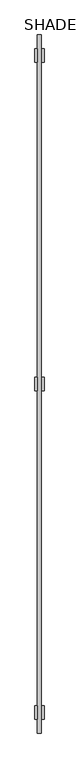
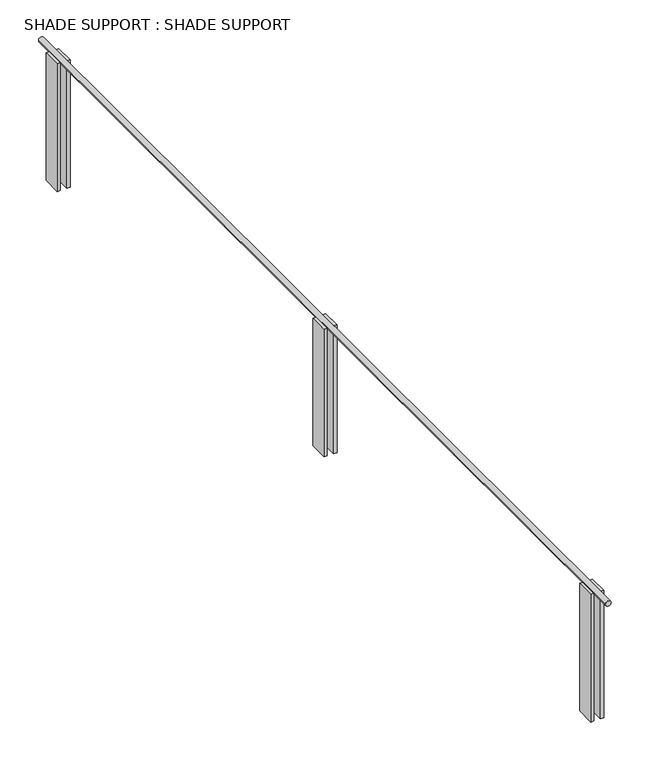
"""IFC4 building model written with IfcOpenShell, lengths in millimetres: proxy geometry, SHADE SUPPORT : SHADE SUPPORT."""

from ifc_helpers import new_model, si_unit, point, frame, frame_2d, origin, origin_with_axes, place, context, project, spatial, polyline, circle_curve, trimmed, segment, composite_curve, outline, extrude, source, transform, mapped, element, save


def shade_support_shade_support_fc9bf8e5(model_context):
    return source(origin(), model_context, "Body", "SweptSolid", [
        extrude(outline(composite_curve([segment(trimmed(circle_curve(frame_2d((1066.8, 0.0)), 22.225), [point((1066.8, -22.225))], [point((1066.8, 22.225))], False, "CARTESIAN"), True, "CONTINUOUS"), segment(trimmed(circle_curve(frame_2d((1066.8, 0.0)), 22.225), [point((1066.8, 22.225))], [point((1066.8, -22.225))], False, "CARTESIAN"), True, "CONTINUOUS")], self_intersect=False)), frame((0.0, -304.8, 0.0), z_axis=(0.0, 1.0, 0.0), x_axis=(0.0, 0.0, 1.0)), (0.0, 0.0, 1.0), 7772.4),
        extrude(outline(polyline([(-25.4, -152.4), (-50.8, -152.4), (-50.8, 0.0), (-25.4, 0.0), (-25.4, -152.4)])), origin_with_axes(), (0.0, 0.0, 1.0), 1066.8),
        extrude(outline(polyline([(50.8, -152.4), (25.4, -152.4), (25.4, 0.0), (50.8, 0.0), (50.8, -152.4)])), origin_with_axes(), (0.0, 0.0, 1.0), 1066.8),
        extrude(outline(polyline([(50.8, 3505.2), (25.4, 3505.2), (25.4, 3657.6), (50.8, 3657.6), (50.8, 3505.2)])), origin_with_axes(), (0.0, 0.0, 1.0), 1066.8),
        extrude(outline(polyline([(-25.4, 3505.2), (-50.8, 3505.2), (-50.8, 3657.6), (-25.4, 3657.6), (-25.4, 3505.2)])), origin_with_axes(), (0.0, 0.0, 1.0), 1066.8),
        extrude(outline(polyline([(50.8, 7162.8), (25.4, 7162.8), (25.4, 7315.2), (50.8, 7315.2), (50.8, 7162.8)])), origin_with_axes(), (0.0, 0.0, 1.0), 1066.8),
        extrude(outline(polyline([(-25.4, 7162.8), (-50.8, 7162.8), (-50.8, 7315.2), (-25.4, 7315.2), (-25.4, 7162.8)])), origin_with_axes(), (0.0, 0.0, 1.0), 1066.8),
    ])


if __name__ == "__main__":
    model = new_model("IFC4")
    model_context = context("Model", 3, world=origin())
    ifc_project = project(units=[si_unit("LENGTHUNIT", "METRE", prefix="MILLI")], contexts=[model_context])
    site = spatial("IfcSite", under=ifc_project)
    building = spatial("IfcBuilding", under=site)
    placement = place(None, origin())
    shade_support_shade_support_shape = shade_support_shade_support_fc9bf8e5(model_context)
    element("IfcBuildingElementProxy", 1, Name="SHADE SUPPORT : SHADE SUPPORT", ObjectType="SHADE SUPPORT : SHADE SUPPORT", at=placement, inside=building, context=model_context, shape_type="MappedRepresentation", body=[
        mapped(shade_support_shade_support_shape, transform((0.0, 0.0, 0.0), x_axis=(1.0, 0.0, 0.0), y_axis=(0.0, 1.0, 0.0), z_axis=(0.0, 0.0, 1.0))),
    ])
    save(model, "model.ifc")

# Revit data of these elements
# Type "SHADE SUPPORT : SHADE SUPPORT"
#   Default Elevation = 12' - 0"
#   DEPTH = 3' - 6"
#   3rd to Roof = 12' - 0"
#   2nd to 3rd = 12' - 0"
#   Assembly Code = ""
# Element 1 (IfcBuildingElementProxy, "SHADE SUPPORT : SHADE SUPPORT")
#   Materials on its faces: "SHADE SUPPORT"
# Materials
#   "SHADE SUPPORT": class "Unassigned", colour RGB 247 247 247, transparency 0
